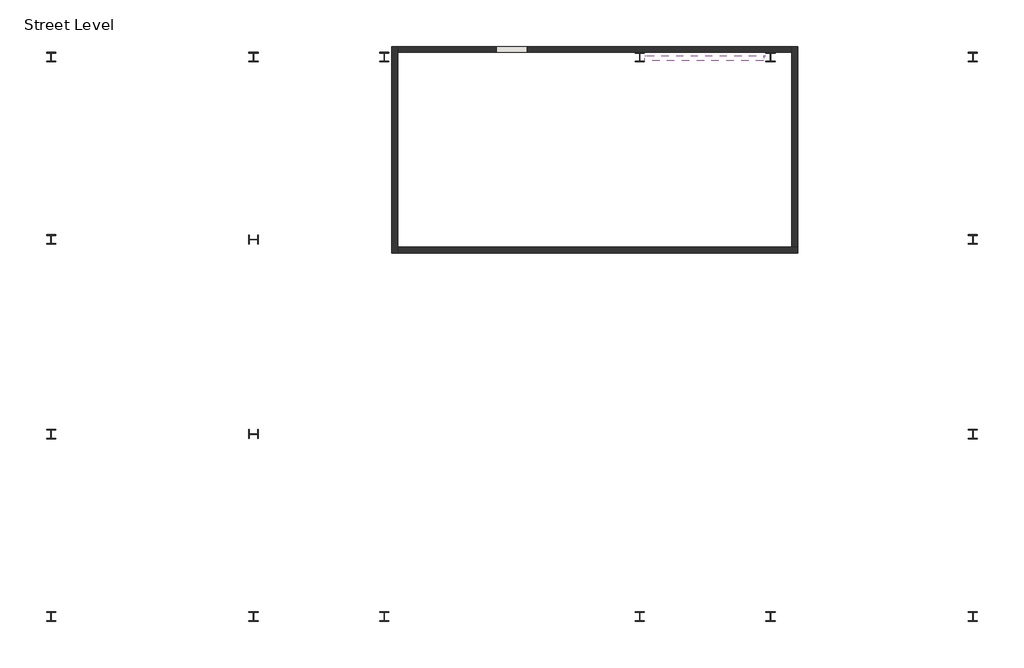
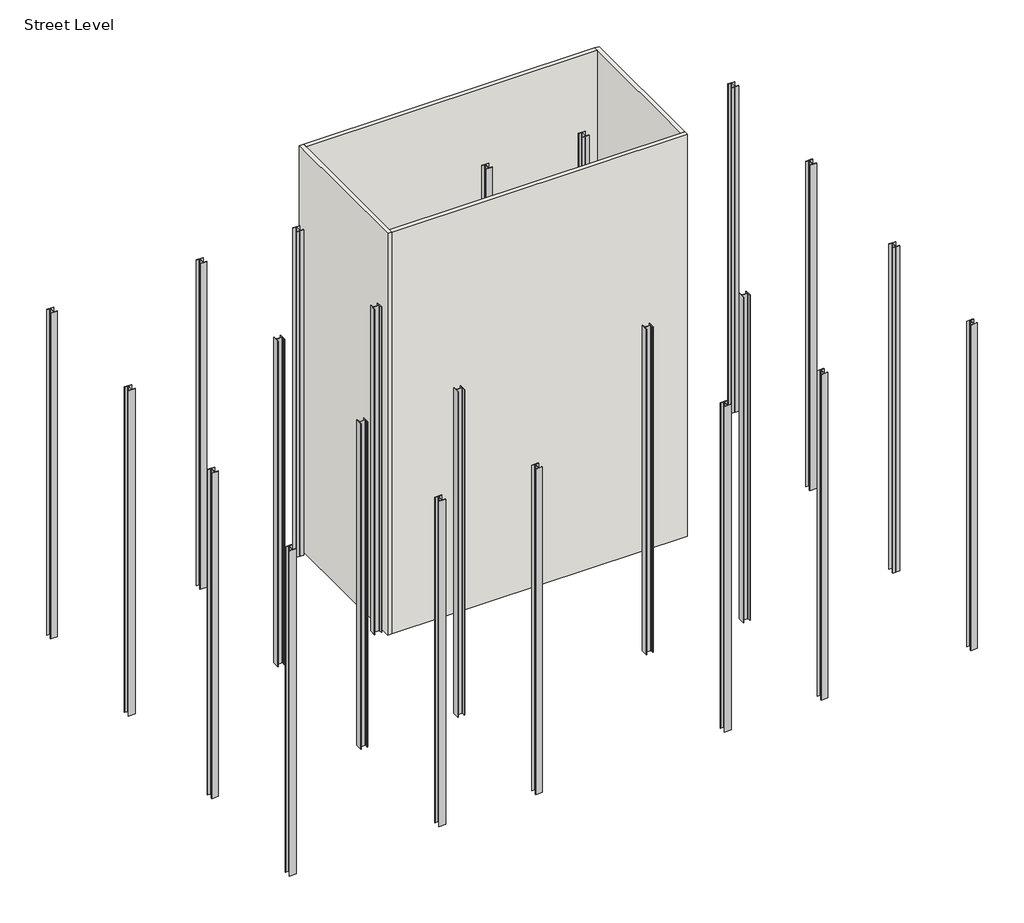
# One storey: 24 columns, 4 walls, 1 member.
"""IFC4 building model written with IfcOpenShell, lengths in millimetres."""

import ifcopenshell
import ifcopenshell.guid

model = None  # the IFC model being written
_history = None  # IfcOwnerHistory: only IFC2X3 demands one
_inside = {}  # id of a spatial element -> (the spatial element, [elements in it])
_under = {}  # id of a project, library or spatial element -> (it, [spatial elements below it])
_declared = {}  # id of a project -> (the project, [libraries it declares])
_typed = {}  # id of a type object -> (the type object, [elements of that type])
_made_of = {}  # id of a material, layer set ... -> (it, [elements and type objects made of it])


def new_model(schema):
    """Start an empty IFC model of exactly this schema.

    Asked for "IFC4X3", IfcOpenShell would pick the latest addendum, in which some entities
    have other attributes; the version numbers below select the first issue.
    IFC2X3 requires an IfcOwnerHistory on every rooted entity: one is made here for all.
    """
    global model, _history
    if schema == "IFC4X3":
        model = ifcopenshell.file(schema_version=(4, 3, 0, 0))
    else:
        model = ifcopenshell.file(schema=schema)
    _inside.clear()
    _under.clear()
    _declared.clear()
    _typed.clear()
    _made_of.clear()
    _history = None
    if model.schema == "IFC2X3":
        org = make("IfcOrganization", Name="unknown")
        user = make(
            "IfcPersonAndOrganization",
            ThePerson=make("IfcPerson", FamilyName="unknown"),
            TheOrganization=org,
        )
        app = make(
            "IfcApplication",
            ApplicationDeveloper=org,
            Version="unknown",
            ApplicationFullName="unknown",
            ApplicationIdentifier="unknown",
        )
        _history = make(
            "IfcOwnerHistory",
            OwningUser=user,
            OwningApplication=app,
            ChangeAction="ADDED",
            CreationDate=0,
        )
    return model


def make(cls, **values):
    """One entity of the class cls with the attributes given. An attribute that is None is left unset."""
    return model.create_entity(
        cls, **{name: value for name, value in values.items() if value is not None}
    )


def rooted(cls, **values):
    """An entity with a GlobalId (a new one), such as an element, a storey or a relation."""
    return make(cls, GlobalId=ifcopenshell.guid.new(), OwnerHistory=_history, **values)


def si_unit(unit_type, name, prefix=None):
    """IfcSIUnit, for example si_unit("LENGTHUNIT", "METRE", prefix="MILLI")."""
    return make("IfcSIUnit", UnitType=unit_type, Prefix=prefix, Name=name)


def assignment(units):
    """IfcUnitAssignment: the units of a project."""
    return None if units is None else make("IfcUnitAssignment", Units=units)


def point(xyz):
    """IfcCartesianPoint."""
    return None if xyz is None else make("IfcCartesianPoint", Coordinates=xyz)


def direction(xyz):
    """IfcDirection."""
    return None if xyz is None else make("IfcDirection", DirectionRatios=xyz)


def frame(location, z_axis=None, x_axis=None):
    """IfcAxis2Placement3D, a coordinate frame: its origin and axes. An axis left out is left unset."""
    return make(
        "IfcAxis2Placement3D",
        Location=point(location),
        Axis=direction(z_axis),
        RefDirection=direction(x_axis),
    )


def frame_2d(location, x_axis=None):
    """IfcAxis2Placement2D, a coordinate frame in the plane: its origin and x axis."""
    return make(
        "IfcAxis2Placement2D", Location=point(location), RefDirection=direction(x_axis)
    )


def origin():
    """The frame at (0, 0, 0) with its axes left unset."""
    return frame((0.0, 0.0, 0.0))


def place(relative_to, where):
    """IfcLocalPlacement: puts the frame where relative to a parent placement (None: the world)."""
    return make(
        "IfcLocalPlacement", PlacementRelTo=relative_to, RelativePlacement=where
    )


def context(
    kind, dimensions, precision=None, world=None, true_north=None, identifier=None
):
    """IfcGeometricRepresentationContext, for example the 3D "Model" context."""
    return make(
        "IfcGeometricRepresentationContext",
        ContextIdentifier=identifier,
        ContextType=kind,
        CoordinateSpaceDimension=dimensions,
        Precision=precision,
        WorldCoordinateSystem=world,
        TrueNorth=true_north,
    )


def project(units=None, contexts=None):
    """IfcProject with its units and contexts."""
    return rooted(
        "IfcProject",
        Name="project",
        RepresentationContexts=contexts,
        UnitsInContext=assignment(units),
    )


def spatial(cls, under=None, at=None, **own):
    """A site, building, storey or space (cls), placed at a placement, below another one or the project."""
    s = rooted(cls, ObjectPlacement=at, **own)
    if under is not None:
        _under.setdefault(under.id(), (under, []))[1].append(s)
    return s


def polyline(points):
    """IfcPolyline through the points."""
    return make("IfcPolyline", Points=[point(p) for p in points])


def circle_curve(where, radius):
    """IfcCircle in the frame where."""
    return make("IfcCircle", Position=where, Radius=radius)


def trimmed(basis, trim1, trim2, sense, master):
    """IfcTrimmedCurve: the piece of a basis curve between two trims."""
    return make(
        "IfcTrimmedCurve",
        BasisCurve=basis,
        Trim1=trim1,
        Trim2=trim2,
        SenseAgreement=sense,
        MasterRepresentation=master,
    )


def segment(curve, same_sense, transition):
    """IfcCompositeCurveSegment."""
    return make(
        "IfcCompositeCurveSegment",
        Transition=transition,
        SameSense=same_sense,
        ParentCurve=curve,
    )


def composite_curve(segments, self_intersect=None):
    """IfcCompositeCurve: segments joined end to end."""
    return make("IfcCompositeCurve", Segments=segments, SelfIntersect=self_intersect)


def outline(outer, holes=None, kind="AREA"):
    """IfcArbitraryClosedProfileDef: a profile drawn as a closed curve; with holes, ...WithVoids."""
    if holes is None:
        return make("IfcArbitraryClosedProfileDef", ProfileType=kind, OuterCurve=outer)
    return make(
        "IfcArbitraryProfileDefWithVoids",
        ProfileType=kind,
        OuterCurve=outer,
        InnerCurves=holes,
    )


def extrude(swept, where, along, depth):
    """IfcExtrudedAreaSolid: the profile swept, set in the frame where, extruded along a direction by depth."""
    return make(
        "IfcExtrudedAreaSolid",
        SweptArea=swept,
        Position=where,
        ExtrudedDirection=direction(along),
        Depth=depth,
    )


def faces_of(points, faces, orient=None, outer=None):
    """IfcFace entities. A face is a list of loops; a loop is a list of indices into points, from 0.

    orient and outer hold one flag for each loop. By default every Orientation is true, the
    first loop of a face is its IfcFaceOuterBound and the others are IfcFaceBound.
    """
    made = []
    for i, loops in enumerate(faces):
        bounds = []
        for j, loop in enumerate(loops):
            is_outer = j == 0 if outer is None else outer[i][j]
            bounds.append(
                make(
                    "IfcFaceOuterBound" if is_outer else "IfcFaceBound",
                    Bound=make("IfcPolyLoop", Polygon=[points[k] for k in loop]),
                    Orientation=True if orient is None else orient[i][j],
                )
            )
        made.append(make("IfcFace", Bounds=bounds))
    return made


def faceted_brep(points, faces, orient=None, outer=None, voids=None):
    """IfcFacetedBrep: a solid bounded by flat faces; with voids (closed shells), ...WithVoids."""
    shared = [point(p) for p in points]
    hull = make("IfcClosedShell", CfsFaces=faces_of(shared, faces, orient, outer))
    if voids is None:
        return make("IfcFacetedBrep", Outer=hull)
    return make(
        "IfcFacetedBrepWithVoids",
        Outer=hull,
        Voids=[
            make(cls, CfsFaces=faces_of(shared, fs, o, b)) for cls, fs, o, b in voids
        ],
    )


def shape(context_of_items, identifier, shape_type, items):
    """IfcShapeRepresentation: the items that make up one representation, for example the "Body"."""
    return make(
        "IfcShapeRepresentation",
        ContextOfItems=context_of_items,
        RepresentationIdentifier=identifier,
        RepresentationType=shape_type,
        Items=items,
    )


def source(mapping_origin, context_of_items, identifier, shape_type, items):
    """IfcRepresentationMap: a shape defined once, which mapped items show again and again."""
    return make(
        "IfcRepresentationMap",
        MappingOrigin=mapping_origin,
        MappedRepresentation=shape(context_of_items, identifier, shape_type, items),
    )


def transform(
    local_origin,
    x_axis=None,
    y_axis=None,
    z_axis=None,
    scale=None,
    scale2=None,
    scale3=None,
    uniform=True,
):
    """IfcCartesianTransformationOperator3D, or its non-uniform kind. x_axis, y_axis, z_axis: its Axis1, 2, 3."""
    if uniform:
        return make(
            "IfcCartesianTransformationOperator3D",
            Axis1=direction(x_axis),
            Axis2=direction(y_axis),
            LocalOrigin=point(local_origin),
            Scale=scale,
            Axis3=direction(z_axis),
        )
    return make(
        "IfcCartesianTransformationOperator3DnonUniform",
        Axis1=direction(x_axis),
        Axis2=direction(y_axis),
        LocalOrigin=point(local_origin),
        Scale=scale,
        Axis3=direction(z_axis),
        Scale2=scale2,
        Scale3=scale3,
    )


def mapped(mapping_source, mapping_target):
    """IfcMappedItem: shows the shape of a source again, moved by a transform."""
    return make(
        "IfcMappedItem", MappingSource=mapping_source, MappingTarget=mapping_target
    )


def made_of(thing, what):
    """Note that an element or type object is made of a material, layer set ...; save() writes the relation."""
    if what is not None:
        _made_of.setdefault(what.id(), (what, []))[1].append(thing)
    return thing


def element(
    cls,
    number,
    at=None,
    inside=None,
    cuts=None,
    type_object=None,
    material=None,
    context=None,
    identifier="Body",
    shape_type=None,
    held_by="IfcProductDefinitionShape",
    body=None,
    shapes=None,
    **own,
):
    """One element of the class cls, such as IfcWall. Its Tag is "e" and its number.

    at: its placement. inside: the storey or other place that contains it. cuts: it is an
    opening in that element (IfcRelVoidsElement). A single representation is given by context,
    identifier, shape_type and body (its items); several are given by shapes. held_by: the class
    of the entity that holds the representations. save() writes the other relations.
    """
    e = rooted(cls, Tag="e%d" % number, ObjectPlacement=at, **own)
    if body is not None:
        shapes = [shape(context, identifier, shape_type, body)]
    if shapes is not None:
        e.Representation = make(held_by, Representations=shapes)
    if inside is not None:
        _inside.setdefault(inside.id(), (inside, []))[1].append(e)
    if cuts is not None:
        rooted(
            "IfcRelVoidsElement", RelatingBuildingElement=cuts, RelatedOpeningElement=e
        )
    if type_object is not None:
        _typed.setdefault(type_object.id(), (type_object, []))[1].append(e)
    return made_of(e, material)


def aggregate(whole, parts):
    """IfcRelAggregates: a whole, such as a stair, and the parts it consists of."""
    return rooted("IfcRelAggregates", RelatingObject=whole, RelatedObjects=parts)


def save(model, path):
    """Write the relations noted so far, then the file.

    IfcRelAggregates (storeys below a building ...), IfcRelContainedInSpatialStructure (elements
    in a storey), IfcRelDefinesByType, IfcRelAssociatesMaterial and IfcRelDeclares: one each for
    every whole, place, type object, material and project.
    """
    for whole, parts in _under.values():
        aggregate(whole, parts)
    for where, things in _inside.values():
        rooted(
            "IfcRelContainedInSpatialStructure",
            RelatedElements=things,
            RelatingStructure=where,
        )
    for kind, things in _typed.values():
        rooted("IfcRelDefinesByType", RelatedObjects=things, RelatingType=kind)
    for what, things in _made_of.values():
        rooted("IfcRelAssociatesMaterial", RelatedObjects=things, RelatingMaterial=what)
    for by, libraries in _declared.values():
        rooted("IfcRelDeclares", RelatingContext=by, RelatedDefinitions=libraries)
    model.write(path)


def w_wide_flange_column_w12x87_da20b1fb(model_context):
    return source(origin(), model_context, "Body", "SweptSolid", [
        extrude(outline(composite_curve([segment(polyline([(153.9875, 159.146875), (153.9875, 138.6085937), (28.8726562, 138.6085937)]), True, "CONTINUOUS"), segment(trimmed(circle_curve(frame_2d((28.8726562, 116.284375)), 22.3242188), [point((28.8726562, 138.6085937))], [point((6.5484375, 116.284375))], True, "CARTESIAN"), True, "CONTINUOUS"), segment(polyline([(6.5484375, 116.284375), (6.5484375, -116.284375)]), True, "CONTINUOUS"), segment(trimmed(circle_curve(frame_2d((28.8726562, -116.284375)), 22.3242188), [point((6.5484375, -116.284375))], [point((28.8726562, -138.6085937))], True, "CARTESIAN"), True, "CONTINUOUS"), segment(polyline([(28.8726562, -138.6085937), (153.9875, -138.6085937), (153.9875, -159.146875), (-153.9875, -159.146875), (-153.9875, -138.6085937), (-28.8726563, -138.6085937)]), True, "CONTINUOUS"), segment(trimmed(circle_curve(frame_2d((-28.8726563, -116.284375)), 22.3242188), [point((-28.8726563, -138.6085937))], [point((-6.5484375, -116.284375))], True, "CARTESIAN"), True, "CONTINUOUS"), segment(polyline([(-6.5484375, -116.284375), (-6.5484375, 116.284375)]), True, "CONTINUOUS"), segment(trimmed(circle_curve(frame_2d((-28.8726563, 116.284375)), 22.3242188), [point((-6.5484375, 116.284375))], [point((-28.8726563, 138.6085937))], True, "CARTESIAN"), True, "CONTINUOUS"), segment(polyline([(-28.8726563, 138.6085937), (-153.9875, 138.6085937), (-153.9875, 159.146875), (153.9875, 159.146875)]), True, "CONTINUOUS")], self_intersect=False)), frame((0.0, 0.0, -914.4), z_axis=(0.0, 0.0, 1.0), x_axis=(1.0, 0.0, 0.0)), (0.0, 0.0, 1.0), 15544.8),
    ])


def l_angle2_l6x6x3_8_34c47d6c(model_context):
    return source(origin(), model_context, "Body", "SweptSolid", [
        extrude(outline(composite_curve([segment(polyline([(41.148, 41.148), (41.148, -111.252)]), True, "CONTINUOUS"), segment(trimmed(circle_curve(frame_2d((41.148, -101.727)), 9.525), [point((41.148, -111.252))], [point((31.623, -101.727))], False, "CARTESIAN"), True, "CONTINUOUS"), segment(polyline([(31.623, -101.727), (31.623, 22.098)]), True, "CONTINUOUS"), segment(trimmed(circle_curve(frame_2d((22.098, 22.098)), 9.525), [point((31.623, 22.098))], [point((22.098, 31.623))], True, "CARTESIAN"), True, "CONTINUOUS"), segment(polyline([(22.098, 31.623), (-101.727, 31.623)]), True, "CONTINUOUS"), segment(trimmed(circle_curve(frame_2d((-101.727, 41.148)), 9.525), [point((-101.727, 31.623))], [point((-111.252, 41.148))], False, "CARTESIAN"), True, "CONTINUOUS"), segment(polyline([(-111.252, 41.148), (41.148, 41.148)]), True, "CONTINUOUS")], self_intersect=False)), frame((-2289.5946037, 0.0, 0.0), z_axis=(1.0, 0.0, 0.0), x_axis=(0.0, 1.0, 0.0)), (0.0, 0.0, 1.0), 4540.0613934),
    ])


model = new_model("IFC4")

# Units and contexts
model_context = context("Model", 3, world=origin())
ifc_project = project(units=[si_unit("LENGTHUNIT", "METRE", prefix="MILLI")], contexts=[model_context])

# Site, building, storey
site = spatial("IfcSite", under=ifc_project)
building = spatial("IfcBuilding", under=site)
storey = spatial("IfcBuildingStorey", under=building, Name="Street Level", Elevation=-914.4)

# Columns
placement = place(None, origin())
w_wide_flange_column_w12x87_shape = w_wide_flange_column_w12x87_da20b1fb(model_context)
element("IfcColumn", 1, ObjectType="W-Wide Flange-Column : W12X87", at=placement, inside=storey, context=model_context, shape_type="MappedRepresentation", body=[
    mapped(w_wide_flange_column_w12x87_shape, transform((-9801.8122732, -3408.4984696, 0.0), x_axis=(0.0, -1.0, 0.0), y_axis=(1.0, 0.0, 0.0), z_axis=(0.0, 0.0, 1.0))),
])
element("IfcColumn", 2, ObjectType="W-Wide Flange-Column : W12X87", at=placement, inside=storey, context=model_context, shape_type="MappedRepresentation", body=[
    mapped(w_wide_flange_column_w12x87_shape, transform((-5433.0122732, -3408.4984696, 0.0), x_axis=(0.0, -1.0, 0.0), y_axis=(1.0, 0.0, 0.0), z_axis=(0.0, 0.0, 1.0))),
])
element("IfcColumn", 3, ObjectType="W-Wide Flange-Column : W12X87", at=placement, inside=storey, context=model_context, shape_type="MappedRepresentation", body=[
    mapped(w_wide_flange_column_w12x87_shape, transform((3101.3877268, -3408.4984696, 0.0), x_axis=(0.0, -1.0, 0.0), y_axis=(1.0, 0.0, 0.0), z_axis=(0.0, 0.0, 1.0))),
])
element("IfcColumn", 4, ObjectType="W-Wide Flange-Column : W12X87", at=placement, inside=storey, context=model_context, shape_type="MappedRepresentation", body=[
    mapped(w_wide_flange_column_w12x87_shape, transform((7470.1877268, -3408.4984696, 0.0), x_axis=(0.0, -1.0, 0.0), y_axis=(1.0, 0.0, 0.0), z_axis=(0.0, 0.0, 1.0))),
])
element("IfcColumn", 5, ObjectType="W-Wide Flange-Column : W12X87", at=placement, inside=storey, context=model_context, shape_type="MappedRepresentation", body=[
    mapped(w_wide_flange_column_w12x87_shape, transform((-9801.8122732, 3093.9015304, 0.0), x_axis=(0.0, -1.0, 0.0), y_axis=(1.0, 0.0, 0.0), z_axis=(0.0, 0.0, 1.0))),
])
element("IfcColumn", 6, ObjectType="W-Wide Flange-Column : W12X87", at=placement, inside=storey, context=model_context, shape_type="MappedRepresentation", body=[
    mapped(w_wide_flange_column_w12x87_shape, transform((-5433.0122732, 3093.9015304, 0.0), x_axis=(0.0, -1.0, 0.0), y_axis=(1.0, 0.0, 0.0), z_axis=(0.0, 0.0, 1.0))),
])
element("IfcColumn", 7, ObjectType="W-Wide Flange-Column : W12X87", at=placement, inside=storey, context=model_context, shape_type="MappedRepresentation", body=[
    mapped(w_wide_flange_column_w12x87_shape, transform((3101.3877268, 3093.9015304, 0.0), x_axis=(0.0, -1.0, 0.0), y_axis=(1.0, 0.0, 0.0), z_axis=(0.0, 0.0, 1.0))),
])
element("IfcColumn", 8, ObjectType="W-Wide Flange-Column : W12X87", at=placement, inside=storey, context=model_context, shape_type="MappedRepresentation", body=[
    mapped(w_wide_flange_column_w12x87_shape, transform((7470.1877268, 3093.9015304, 0.0), x_axis=(0.0, -1.0, 0.0), y_axis=(1.0, 0.0, 0.0), z_axis=(0.0, 0.0, 1.0))),
])
element("IfcColumn", 9, ObjectType="W-Wide Flange-Column : W12X87", at=placement, inside=storey, context=model_context, shape_type="MappedRepresentation", body=[
    mapped(w_wide_flange_column_w12x87_shape, transform((-16558.2122732, 9189.9015304, 0.0), x_axis=(1.0, 0.0, 0.0), y_axis=(0.0, 1.0, 0.0), z_axis=(0.0, 0.0, 1.0))),
])
element("IfcColumn", 10, ObjectType="W-Wide Flange-Column : W12X87", at=placement, inside=storey, context=model_context, shape_type="MappedRepresentation", body=[
    mapped(w_wide_flange_column_w12x87_shape, transform((-16558.2122732, 3093.9015304, 0.0), x_axis=(1.0, 0.0, 0.0), y_axis=(0.0, 1.0, 0.0), z_axis=(0.0, 0.0, 1.0))),
])
element("IfcColumn", 11, ObjectType="W-Wide Flange-Column : W12X87", at=placement, inside=storey, context=model_context, shape_type="MappedRepresentation", body=[
    mapped(w_wide_flange_column_w12x87_shape, transform((-9801.8122732, 9189.9015304, 0.0), x_axis=(1.0, 0.0, 0.0), y_axis=(0.0, 1.0, 0.0), z_axis=(0.0, 0.0, 1.0))),
])
element("IfcColumn", 12, ObjectType="W-Wide Flange-Column : W12X87", at=placement, inside=storey, context=model_context, shape_type="MappedRepresentation", body=[
    mapped(w_wide_flange_column_w12x87_shape, transform((-5433.0122732, 9189.9015304, 0.0), x_axis=(1.0, 0.0, 0.0), y_axis=(0.0, 1.0, 0.0), z_axis=(0.0, 0.0, 1.0))),
])
element("IfcColumn", 13, ObjectType="W-Wide Flange-Column : W12X87", at=placement, inside=storey, context=model_context, shape_type="MappedRepresentation", body=[
    mapped(w_wide_flange_column_w12x87_shape, transform((3101.3877268, 9189.9015304, 0.0), x_axis=(1.0, 0.0, 0.0), y_axis=(0.0, 1.0, 0.0), z_axis=(0.0, 0.0, 1.0))),
])
element("IfcColumn", 14, ObjectType="W-Wide Flange-Column : W12X87", at=placement, inside=storey, context=model_context, shape_type="MappedRepresentation", body=[
    mapped(w_wide_flange_column_w12x87_shape, transform((7470.1877268, 9189.9015304, 0.0), x_axis=(1.0, 0.0, 0.0), y_axis=(0.0, 1.0, 0.0), z_axis=(0.0, 0.0, 1.0))),
])
element("IfcColumn", 15, ObjectType="W-Wide Flange-Column : W12X87", at=placement, inside=storey, context=model_context, shape_type="MappedRepresentation", body=[
    mapped(w_wide_flange_column_w12x87_shape, transform((14226.5877268, 9189.9015304, 0.0), x_axis=(1.0, 0.0, 0.0), y_axis=(0.0, 1.0, 0.0), z_axis=(0.0, 0.0, 1.0))),
])
element("IfcColumn", 16, ObjectType="W-Wide Flange-Column : W12X87", at=placement, inside=storey, context=model_context, shape_type="MappedRepresentation", body=[
    mapped(w_wide_flange_column_w12x87_shape, transform((14226.5877268, 3093.9015304, 0.0), x_axis=(1.0, 0.0, 0.0), y_axis=(0.0, 1.0, 0.0), z_axis=(0.0, 0.0, 1.0))),
])
element("IfcColumn", 17, ObjectType="W-Wide Flange-Column : W12X87", at=placement, inside=storey, context=model_context, shape_type="MappedRepresentation", body=[
    mapped(w_wide_flange_column_w12x87_shape, transform((14226.5877268, -3408.4984696, 0.0), x_axis=(1.0, 0.0, 0.0), y_axis=(0.0, 1.0, 0.0), z_axis=(0.0, 0.0, 1.0))),
])
element("IfcColumn", 18, ObjectType="W-Wide Flange-Column : W12X87", at=placement, inside=storey, context=model_context, shape_type="MappedRepresentation", body=[
    mapped(w_wide_flange_column_w12x87_shape, transform((14226.5877268, -9504.4984696, 0.0), x_axis=(1.0, 0.0, 0.0), y_axis=(0.0, 1.0, 0.0), z_axis=(0.0, 0.0, 1.0))),
])
element("IfcColumn", 19, ObjectType="W-Wide Flange-Column : W12X87", at=placement, inside=storey, context=model_context, shape_type="MappedRepresentation", body=[
    mapped(w_wide_flange_column_w12x87_shape, transform((7470.1877268, -9504.4984696, 0.0), x_axis=(1.0, 0.0, 0.0), y_axis=(0.0, 1.0, 0.0), z_axis=(0.0, 0.0, 1.0))),
])
element("IfcColumn", 20, ObjectType="W-Wide Flange-Column : W12X87", at=placement, inside=storey, context=model_context, shape_type="MappedRepresentation", body=[
    mapped(w_wide_flange_column_w12x87_shape, transform((3101.3877268, -9504.4984696, 0.0), x_axis=(1.0, 0.0, 0.0), y_axis=(0.0, 1.0, 0.0), z_axis=(0.0, 0.0, 1.0))),
])
element("IfcColumn", 21, ObjectType="W-Wide Flange-Column : W12X87", at=placement, inside=storey, context=model_context, shape_type="MappedRepresentation", body=[
    mapped(w_wide_flange_column_w12x87_shape, transform((-5433.0122732, -9504.4984696, 0.0), x_axis=(1.0, 0.0, 0.0), y_axis=(0.0, 1.0, 0.0), z_axis=(0.0, 0.0, 1.0))),
])
element("IfcColumn", 22, ObjectType="W-Wide Flange-Column : W12X87", at=placement, inside=storey, context=model_context, shape_type="MappedRepresentation", body=[
    mapped(w_wide_flange_column_w12x87_shape, transform((-9801.8122732, -9504.4984696, 0.0), x_axis=(1.0, 0.0, 0.0), y_axis=(0.0, 1.0, 0.0), z_axis=(0.0, 0.0, 1.0))),
])
element("IfcColumn", 23, ObjectType="W-Wide Flange-Column : W12X87", at=placement, inside=storey, context=model_context, shape_type="MappedRepresentation", body=[
    mapped(w_wide_flange_column_w12x87_shape, transform((-16558.2122732, -9504.4984696, 0.0), x_axis=(1.0, 0.0, 0.0), y_axis=(0.0, 1.0, 0.0), z_axis=(0.0, 0.0, 1.0))),
])
element("IfcColumn", 24, ObjectType="W-Wide Flange-Column : W12X87", at=placement, inside=storey, context=model_context, shape_type="MappedRepresentation", body=[
    mapped(w_wide_flange_column_w12x87_shape, transform((-16558.2122732, -3408.4984696, 0.0), x_axis=(1.0, 0.0, 0.0), y_axis=(0.0, 1.0, 0.0), z_axis=(0.0, 0.0, 1.0))),
])

# Member
l_angle2_l6x6x3_8_shape = l_angle2_l6x6x3_8_34c47d6c(model_context)
element("IfcMember", 25, ObjectType="L-Angle2 : L6X6X3/8", at=placement, inside=storey, context=model_context, shape_type="MappedRepresentation", body=[
    mapped(l_angle2_l6x6x3_8_shape, transform((5285.7877268, 9189.9015304, 1828.8), x_axis=(0.8731977020149078, 0.0, 0.4873661592641457), y_axis=(0.0, 1.0000000000000002, 0.0), z_axis=(-0.4873661592641457, 0.0, 0.8731977020149078))),
])

# Walls
element("IfcWall", 26, ObjectType="Generic - 8\" Masonry", at=placement, inside=storey, context=model_context, shape_type="Brep", body=[
    faceted_brep([(-5174.2497732, 9545.5015304, -914.4), (-5174.2497732, 2641.4640304, -914.4), (-5174.2497732, 2641.4640304, 18288.0), (-5174.2497732, 9545.5015304, 18288.0), (-4980.5747732, 9545.5015304, -914.4), (-4980.5747732, 9545.5015304, 18288.0), (-4980.5747732, 9351.8265304, 18288.0), (-4980.5747732, 2835.1390304, 18288.0), (-4980.5747732, 2641.4640304, 18288.0), (-4980.5747732, 2641.4640304, -914.4), (-4980.5747732, 2835.1390304, -914.4), (-4980.5747732, 9351.8265304, -914.4)], [[[0, 1, 2, 3]], [[4, 5, 6, 7, 8, 9, 10, 11]], [[1, 0, 4, 11, 10, 9]], [[3, 2, 8, 7, 6, 5]], [[2, 1, 9, 8]], [[0, 3, 5, 4]]]),
])
element("IfcWall", 27, ObjectType="Generic - 8\" Masonry", at=placement, inside=storey, context=model_context, shape_type="Brep", body=[
    faceted_brep([(8379.8252268, 2835.1390304, -914.4), (8186.1502268, 2835.1390304, -914.4), (-4980.5747732, 2835.1390304, -914.4), (-4980.5747732, 2835.1390304, 18288.0), (8186.1502268, 2835.1390304, 18288.0), (8379.8252268, 2835.1390304, 18288.0), (8379.8252268, 2641.4640304, -914.4), (8379.8252268, 2641.4640304, 18288.0), (-4980.5747732, 2641.4640304, 18288.0), (-4980.5747732, 2641.4640304, -914.4)], [[[0, 1, 2, 3, 4, 5]], [[6, 7, 8, 9]], [[2, 1, 0, 6, 9]], [[5, 4, 3, 8, 7]], [[0, 5, 7, 6]], [[3, 2, 9, 8]]]),
])
element("IfcWall", 28, ObjectType="Generic - 8\" Masonry", at=placement, inside=storey, context=model_context, shape_type="Brep", body=[
    faceted_brep([(8186.1502268, 9545.5015304, -914.4), (8186.1502268, 9351.8265304, -914.4), (8186.1502268, 2835.1390304, -914.4), (8186.1502268, 2835.1390304, 18288.0), (8186.1502268, 9351.8265304, 18288.0), (8186.1502268, 9545.5015304, 18288.0), (8379.8252268, 9545.5015304, -914.4), (8379.8252268, 9545.5015304, 18288.0), (8379.8252268, 2835.1390304, 18288.0), (8379.8252268, 2835.1390304, -914.4)], [[[0, 1, 2, 3, 4, 5]], [[6, 7, 8, 9]], [[2, 1, 0, 6, 9]], [[5, 4, 3, 8, 7]], [[0, 5, 7, 6]], [[3, 2, 9, 8]]]),
])
element("IfcWall", 29, ObjectType="Generic - 8\" Masonry", at=placement, inside=storey, context=model_context, shape_type="SweptSolid", body=[
    extrude(outline(polyline([(-914.4, -4980.5747732), (-914.4, 8186.1502268), (18288.0, 8186.1502268), (18288.0, -4980.5747732), (-914.4, -4980.5747732)]), holes=[polyline([(2235.2, -1692.8622732), (2235.2, -657.8122732), (0.0, -657.8122732), (0.0, -1692.8622732), (2235.2, -1692.8622732)])]), frame((0.0, 9351.8265304, 0.0), z_axis=(0.0, 1.0, 0.0), x_axis=(0.0, 0.0, 1.0)), (0.0, 0.0, 1.0), 193.675),
])

save(model, "model.ifc")

# Revit data of these elements
# Project information
#   Organization Name = "G3B Press"
#   Organization Description = "Paul F. Aubin Cosulting Services, Inc."
#   Building Name = "Revit Essentials for Architecture"
#   Author = "Paul F. Aubin"
#   Author Website = "https://www.paulaubin.com"
#   Copyright = "Copyright © 2020 Paul F Aubin, all rights reserved"
#   Project Issue Date = "8/1/2020"
#   Project Status = "Design Development"
#   Client Name = "Vertical Circulation"
#   Project Address = "123 State ST\nSuite 301\nChicago, IL 60606"
#   Project Name = "08 Commercial-Structure"
#   Project Number = "2020.04S"
# Grids (mm)
#   "1": line (-22547.601, -9504.498) -> (19277.595, -9504.498)
#   "2": line (-22547.601, -3408.498) -> (19277.595, -3408.498)
#   "3": line (-22547.601, 3093.902) -> (19277.595, 3093.902)
#   "4": line (-22547.601, 9189.902) -> (19277.595, 9189.902)
#   "A": line (-16558.212, 12259.726) -> (-16558.212, -14197.104)
#   "B": line (-9801.812, 12259.726) -> (-9801.812, -14197.104)
#   "C": line (-5433.012, 12259.726) -> (-5433.012, -14197.104)
#   "D": line (3101.388, 12259.726) -> (3101.388, -14197.104)
#   "E": line (7470.188, 12259.726) -> (7470.188, -14197.104)
#   "F": line (14226.588, 12259.726) -> (14226.588, -14197.104)
#   "C.3": line (-2689.812, -15151.11) -> (-2689.812, -5965.346)
#   "C.7": line (358.188, -15151.11) -> (358.188, -5965.346)
# Type "W-Wide Flange-Column : W12X87"
#   Assembly Code = "B10"
#   A = 0.18 SF
#   W = 87
#   bf = 1' - 0 1/8"
#   d = 1' - 0 17/32"
#   k = 0' - 1 11/16"
#   kr = 0' - 0 225/256"
#   tf = 0' - 0 207/256"
#   tw = 0' - 0 33/64"
#   Structural Material [instance default] = Metal - Steel - ASTM A992
# Type "L-Angle2 : L6X6X3/8"
#   Assembly Code = "B10"
#   k = 0' - 0 7/8"
#   W = 14.9
#   Length [instance default] = 5' - 0"
#   b = 0' - 6"
#   d = 0' - 6"
#   t = 0' - 0 3/8"
#   x = 0' - 1.62"
#   y = 0' - 1.62"
#   A = 0.0304167 SF
#   Structural Material [instance default] = Steel ASTM A36
# Type "Generic - 8\" Masonry"
#   Assembly Code = "B2010"
#   Layers, outside or top first: 0' - 7 5/8" "Masonry - Concrete Masonry Units" (function 1)
# Elements 1, 2, 3, 4, 5, 6, 7, 8, 9, 10, 11, 12, 13, 14, 15, 16, 17, 18, 19, 20, 21, 22, 23, 24 (IfcColumn, "W-Wide Flange-Column : W12X87")
#   Structural Material = Metal - Steel - ASTM A992
#   Phase Created = New Construction
#   Materials on its faces: "Metal - Steel - ASTM A992"
# Element 25 (IfcMember, "L-Angle2 : L6X6X3/8")
#   Structural Material = Steel ASTM A36
#   Phase Created = New Construction
#   Materials on its faces: "Steel ASTM A36"
# Elements 26, 27, 28, 29 (IfcWall, "Generic - 8\" Masonry")
#   Top Offset = 12' - 0"
#   Base Offset = 0' - 0"
#   Unconnected Height = 63' - 0"
#   wall height = 63' - 0"
#   Phase Created = New Construction
#   Base Constraint = Street Level
#   Top Constraint = Roof
#   Materials on its faces: "Masonry - Concrete Masonry Units"
# Materials
#   "Metal - Steel - ASTM A992": class "Unassigned", colour RGB 199 199 199, transparency 0, Description = "Steel ASTM A992"
#   "Steel ASTM A36": class "Metal", colour RGB 199 199 199, transparency 0, Description = "Structural steel, ASTM A36 Grade B, mill finish", Cost = 0
#   "Masonry - Concrete Masonry Units": class "Unassigned", colour RGB 227 227 227, transparency 0, Description = "CMU"
